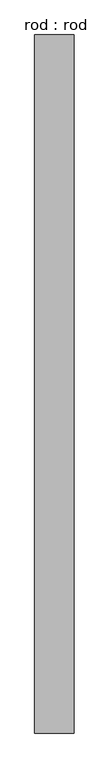
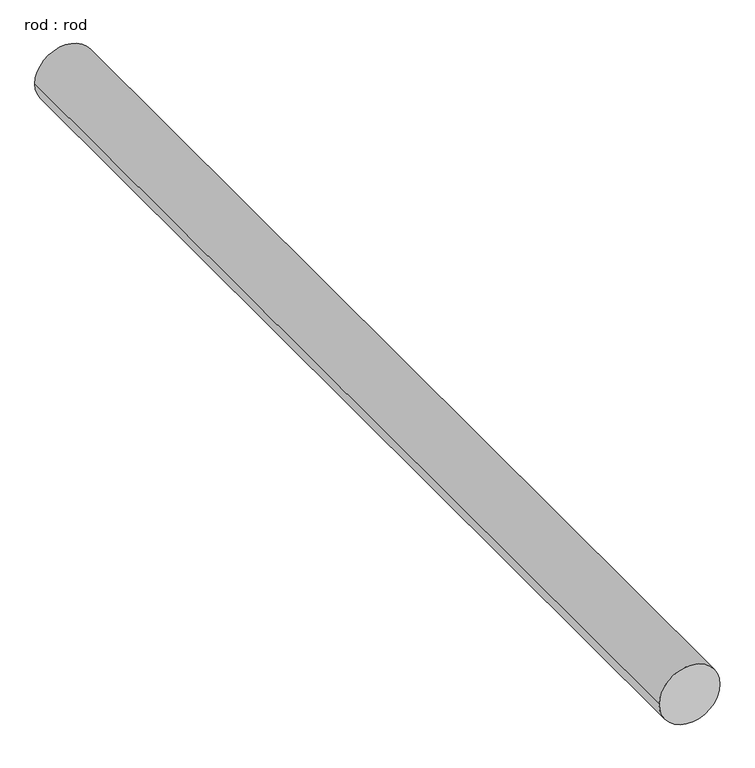
"""IFC4 building model written with IfcOpenShell, lengths in millimetres: proxy geometry, rod : rod."""

from ifc_helpers import new_model, si_unit, point, frame, frame_2d, origin, place, context, project, spatial, circle_curve, trimmed, segment, composite_curve, outline, extrude, source, transform, mapped, element, save


def rod_rod_88a5e3f3(model_context):
    return source(origin(), model_context, "Body", "SweptSolid", [
        extrude(outline(composite_curve([segment(trimmed(circle_curve(frame_2d((0.0108462, 0.0)), 200.0), [point((0.0108462, 200.0))], [point((0.0108462, -200.0))], False, "CARTESIAN"), True, "CONTINUOUS"), segment(trimmed(circle_curve(frame_2d((0.0108462, 0.0)), 200.0), [point((0.0108462, -200.0))], [point((0.0108462, 200.0))], False, "CARTESIAN"), True, "CONTINUOUS")], self_intersect=False)), frame((0.0, 530.8953015, 0.0), z_axis=(0.0, 1.0, 0.0), x_axis=(0.0, 0.0, 1.0)), (0.0, 0.0, 1.0), 7123.6666277),
    ])


if __name__ == "__main__":
    model = new_model("IFC4")
    model_context = context("Model", 3, world=origin())
    ifc_project = project(units=[si_unit("LENGTHUNIT", "METRE", prefix="MILLI")], contexts=[model_context])
    site = spatial("IfcSite", under=ifc_project)
    building = spatial("IfcBuilding", under=site)
    placement = place(None, origin())
    rod_rod_shape = rod_rod_88a5e3f3(model_context)
    element("IfcBuildingElementProxy", 1, Name="rod : rod", ObjectType="rod : rod", at=placement, inside=building, context=model_context, shape_type="MappedRepresentation", body=[
        mapped(rod_rod_shape, transform((0.0, 0.0, 0.0), x_axis=(1.0, 0.0, 0.0), y_axis=(0.0, 1.0, 0.0), z_axis=(0.0, 0.0, 1.0))),
    ])
    save(model, "model.ifc")

# Revit data of these elements
# Type "rod : rod"
#   Default Elevation = 0
